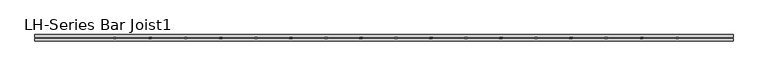
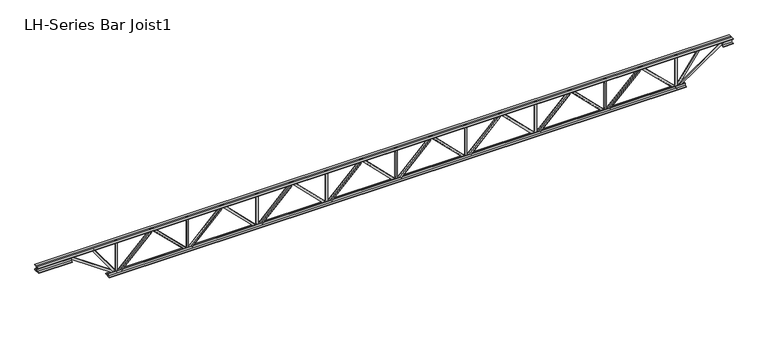
"""IFC4 building model written with IfcOpenShell, lengths in millimetres: beam geometry, LH-Series Bar Joist1 : 32LH-SP5."""

from ifc_helpers import new_model, si_unit, frame, origin, place, context, project, spatial, polyline, outline, extrude, faceted_brep, source, transform, mapped, element, save


def lh_series_bar_joist1_a0e3509c(model_context):
    return source(origin(), model_context, "Body", "SolidModel", [
        extrude(outline(polyline([(406.4, 3276.6), (406.4, 3225.8), (323.85, 3225.8), (312.7375, 3236.9125), (-312.7375, 3236.9125), (-323.85, 3225.8), (-406.4, 3225.8), (-406.4, 3276.6), (406.4, 3276.6)])), frame((0.0, -12.7, 0.0), z_axis=(0.0, 1.0, 0.0), x_axis=(0.0, 0.0, 1.0)), (0.0, 0.0, 1.0), 25.4),
        faceted_brep([(3251.2, 0.0, -355.6), (3251.2, 0.0, -406.4), (3251.2, 12.7, -406.4), (3251.2, 12.7, -355.6), (3236.3210245, 0.0, -355.6), (2474.3210245, 0.0, 406.4), (2413.0, 0.0, 406.4), (2413.0, 0.0, 355.6), (2453.2789755, 0.0, 355.6), (3215.2789755, 0.0, -406.4), (3215.2789755, 12.7, -406.4), (3151.7789755, 12.7, -342.9), (3160.7592316, 12.7, -333.9197439), (2474.9592316, 12.7, 351.8802561), (2465.9789755, 12.7, 342.9), (2453.2789755, 12.7, 355.6), (2413.0, 12.7, 355.6), (2413.0, 12.7, 406.4), (2474.3210245, 12.7, 406.4), (3236.3210245, 12.7, -355.6), (2465.9789755, 50.8, 342.9), (3151.7789755, 50.8, -342.9), (3160.7592316, 50.8, -333.9197439), (2474.9592316, 50.8, 351.8802561)], [[[0, 1, 2, 3]], [[1, 0, 4, 5, 6, 7, 8, 9]], [[2, 1, 9, 10]], [[3, 2, 10, 11, 12, 13, 14, 15, 16, 17, 18, 19]], [[0, 3, 19, 4]], [[9, 8, 15, 14, 20, 21, 11, 10]], [[5, 4, 19, 18]], [[7, 6, 17, 16]], [[8, 7, 16, 15]], [[6, 5, 18, 17]], [[11, 21, 22, 12]], [[13, 23, 20, 14]], [[22, 21, 20, 23]], [[12, 22, 23, 13]]]),
        faceted_brep([(1625.6, -12.7, -355.6), (1625.6, 0.0, -355.6), (1625.6, 0.0, -406.4), (1625.6, -12.7, -406.4), (1640.4789755, -12.7, -355.6), (1640.4789755, 0.0, -355.6), (2402.4789755, 0.0, 406.4), (2463.8, 0.0, 406.4), (2463.8, 0.0, 355.6), (2423.5210245, 0.0, 355.6), (1661.5210245, 0.0, -406.4), (1661.5210245, -12.7, -406.4), (1725.0210245, -12.7, -342.9), (1716.0407684, -12.7, -333.9197439), (2401.8407684, -12.7, 351.8802561), (2410.8210245, -12.7, 342.9), (2423.5210245, -12.7, 355.6), (2463.8, -12.7, 355.6), (2463.8, -12.7, 406.4), (2402.4789755, -12.7, 406.4), (2410.8210245, -50.8, 342.9), (1725.0210245, -50.8, -342.9), (1716.0407684, -50.8, -333.9197439), (2401.8407684, -50.8, 351.8802561)], [[[0, 1, 2, 3]], [[1, 0, 4, 5]], [[2, 1, 5, 6, 7, 8, 9, 10]], [[3, 2, 10, 11]], [[0, 3, 11, 12, 13, 14, 15, 16, 17, 18, 19, 4]], [[5, 4, 19, 6]], [[10, 9, 16, 15, 20, 21, 12, 11]], [[8, 7, 18, 17]], [[7, 6, 19, 18]], [[9, 8, 17, 16]], [[21, 22, 13, 12]], [[20, 15, 14, 23]], [[22, 21, 20, 23]], [[13, 22, 23, 14]]]),
        extrude(outline(polyline([(406.4, 1651.0), (406.4, 1600.2), (323.85, 1600.2), (312.7375, 1611.3125), (-312.7375, 1611.3125), (-323.85, 1600.2), (-406.4, 1600.2), (-406.4, 1651.0), (406.4, 1651.0)])), frame((0.0, -12.7, 0.0), z_axis=(0.0, 1.0, 0.0), x_axis=(0.0, 0.0, 1.0)), (0.0, 0.0, 1.0), 25.4),
        faceted_brep([(1625.6, 0.0, -355.6), (1625.6, 0.0, -406.4), (1625.6, 12.7, -406.4), (1625.6, 12.7, -355.6), (1610.7210245, 0.0, -355.6), (848.7210245, 0.0, 406.4), (787.4, 0.0, 406.4), (787.4, 0.0, 355.6), (827.6789755, 0.0, 355.6), (1589.6789755, 0.0, -406.4), (1589.6789755, 12.7, -406.4), (1526.1789755, 12.7, -342.9), (1535.1592316, 12.7, -333.9197439), (849.3592316, 12.7, 351.8802561), (840.3789755, 12.7, 342.9), (827.6789755, 12.7, 355.6), (787.4, 12.7, 355.6), (787.4, 12.7, 406.4), (848.7210245, 12.7, 406.4), (1610.7210245, 12.7, -355.6), (840.3789755, 50.8, 342.9), (1526.1789755, 50.8, -342.9), (1535.1592316, 50.8, -333.9197439), (849.3592316, 50.8, 351.8802561)], [[[0, 1, 2, 3]], [[1, 0, 4, 5, 6, 7, 8, 9]], [[2, 1, 9, 10]], [[3, 2, 10, 11, 12, 13, 14, 15, 16, 17, 18, 19]], [[0, 3, 19, 4]], [[9, 8, 15, 14, 20, 21, 11, 10]], [[5, 4, 19, 18]], [[7, 6, 17, 16]], [[8, 7, 16, 15]], [[6, 5, 18, 17]], [[11, 21, 22, 12]], [[13, 23, 20, 14]], [[22, 21, 20, 23]], [[12, 22, 23, 13]]]),
        faceted_brep([(0.0, -12.7, -355.6), (0.0, 0.0, -355.6), (0.0, 0.0, -406.4), (0.0, -12.7, -406.4), (14.8789755, -12.7, -355.6), (14.8789755, 0.0, -355.6), (776.8789755, 0.0, 406.4), (838.2, 0.0, 406.4), (838.2, 0.0, 355.6), (797.9210245, 0.0, 355.6), (35.9210245, 0.0, -406.4), (35.9210245, -12.7, -406.4), (99.4210245, -12.7, -342.9), (90.4407684, -12.7, -333.9197439), (776.2407684, -12.7, 351.8802561), (785.2210245, -12.7, 342.9), (797.9210245, -12.7, 355.6), (838.2, -12.7, 355.6), (838.2, -12.7, 406.4), (776.8789755, -12.7, 406.4), (785.2210245, -50.8, 342.9), (99.4210245, -50.8, -342.9), (90.4407684, -50.8, -333.9197439), (776.2407684, -50.8, 351.8802561)], [[[0, 1, 2, 3]], [[1, 0, 4, 5]], [[2, 1, 5, 6, 7, 8, 9, 10]], [[3, 2, 10, 11]], [[0, 3, 11, 12, 13, 14, 15, 16, 17, 18, 19, 4]], [[5, 4, 19, 6]], [[10, 9, 16, 15, 20, 21, 12, 11]], [[8, 7, 18, 17]], [[7, 6, 19, 18]], [[9, 8, 17, 16]], [[21, 22, 13, 12]], [[20, 15, 14, 23]], [[22, 21, 20, 23]], [[13, 22, 23, 14]]]),
        extrude(outline(polyline([(406.4, 25.4), (406.4, -25.4), (323.85, -25.4), (312.7375, -14.2875), (-312.7375, -14.2875), (-323.85, -25.4), (-406.4, -25.4), (-406.4, 25.4), (406.4, 25.4)])), frame((0.0, -12.7, 0.0), z_axis=(0.0, 1.0, 0.0), x_axis=(0.0, 0.0, 1.0)), (0.0, 0.0, 1.0), 25.4),
        faceted_brep([(0.0, 0.0, -355.6), (0.0, 0.0, -406.4), (0.0, 12.7, -406.4), (0.0, 12.7, -355.6), (-14.8789755, 0.0, -355.6), (-776.8789755, 0.0, 406.4), (-838.2, 0.0, 406.4), (-838.2, 0.0, 355.6), (-797.9210245, 0.0, 355.6), (-35.9210245, 0.0, -406.4), (-35.9210245, 12.7, -406.4), (-99.4210245, 12.7, -342.9), (-90.4407684, 12.7, -333.9197439), (-776.2407684, 12.7, 351.8802561), (-785.2210245, 12.7, 342.9), (-797.9210245, 12.7, 355.6), (-838.2, 12.7, 355.6), (-838.2, 12.7, 406.4), (-776.8789755, 12.7, 406.4), (-14.8789755, 12.7, -355.6), (-785.2210245, 50.8, 342.9), (-99.4210245, 50.8, -342.9), (-90.4407684, 50.8, -333.9197439), (-776.2407684, 50.8, 351.8802561)], [[[0, 1, 2, 3]], [[1, 0, 4, 5, 6, 7, 8, 9]], [[2, 1, 9, 10]], [[3, 2, 10, 11, 12, 13, 14, 15, 16, 17, 18, 19]], [[0, 3, 19, 4]], [[9, 8, 15, 14, 20, 21, 11, 10]], [[5, 4, 19, 18]], [[7, 6, 17, 16]], [[8, 7, 16, 15]], [[6, 5, 18, 17]], [[11, 21, 22, 12]], [[13, 23, 20, 14]], [[22, 21, 20, 23]], [[12, 22, 23, 13]]]),
        faceted_brep([(-1625.6, -12.7, -355.6), (-1625.6, 0.0, -355.6), (-1625.6, 0.0, -406.4), (-1625.6, -12.7, -406.4), (-1610.7210245, -12.7, -355.6), (-1610.7210245, 0.0, -355.6), (-848.7210245, 0.0, 406.4), (-787.4, 0.0, 406.4), (-787.4, 0.0, 355.6), (-827.6789755, 0.0, 355.6), (-1589.6789755, 0.0, -406.4), (-1589.6789755, -12.7, -406.4), (-1526.1789755, -12.7, -342.9), (-1535.1592316, -12.7, -333.9197439), (-849.3592316, -12.7, 351.8802561), (-840.3789755, -12.7, 342.9), (-827.6789755, -12.7, 355.6), (-787.4, -12.7, 355.6), (-787.4, -12.7, 406.4), (-848.7210245, -12.7, 406.4), (-840.3789755, -50.8, 342.9), (-1526.1789755, -50.8, -342.9), (-1535.1592316, -50.8, -333.9197439), (-849.3592316, -50.8, 351.8802561)], [[[0, 1, 2, 3]], [[1, 0, 4, 5]], [[2, 1, 5, 6, 7, 8, 9, 10]], [[3, 2, 10, 11]], [[0, 3, 11, 12, 13, 14, 15, 16, 17, 18, 19, 4]], [[5, 4, 19, 6]], [[10, 9, 16, 15, 20, 21, 12, 11]], [[8, 7, 18, 17]], [[7, 6, 19, 18]], [[9, 8, 17, 16]], [[21, 22, 13, 12]], [[20, 15, 14, 23]], [[22, 21, 20, 23]], [[13, 22, 23, 14]]]),
        extrude(outline(polyline([(406.4, 6556.375), (406.4, 6505.575), (323.85, 6505.575), (312.7375, 6516.6875), (-312.7375, 6516.6875), (-323.85, 6505.575), (-406.4, 6505.575), (-406.4, 6556.375), (406.4, 6556.375)])), frame((0.0, -12.7, 0.0), z_axis=(0.0, 1.0, 0.0), x_axis=(0.0, 0.0, 1.0)), (0.0, 0.0, 1.0), 25.4),
        faceted_brep([(6530.975, 0.0, -355.6), (6530.975, 0.0, -406.4), (6530.975, 12.7, -406.4), (6530.975, 12.7, -355.6), (6515.958098, 0.0, -355.6), (5739.670598, 0.0, 406.4), (5678.4875, 0.0, 406.4), (5678.4875, 0.0, 355.6), (5718.904402, 0.0, 355.6), (6495.191902, 0.0, -406.4), (6495.191902, 12.7, -406.4), (6431.104883, 12.7, -343.4924966), (6440.0013474, 12.7, -334.4292234), (5740.6182703, 12.7, 352.0817725), (5731.7218059, 12.7, 343.0184993), (5718.904402, 12.7, 355.6), (5678.4875, 12.7, 355.6), (5678.4875, 12.7, 406.4), (5739.670598, 12.7, 406.4), (6515.958098, 12.7, -355.6), (5731.7218059, 50.8, 343.0184993), (6431.104883, 50.8, -343.4924966), (6440.0013474, 50.8, -334.4292234), (5740.6182703, 50.8, 352.0817725)], [[[0, 1, 2, 3]], [[1, 0, 4, 5, 6, 7, 8, 9]], [[2, 1, 9, 10]], [[3, 2, 10, 11, 12, 13, 14, 15, 16, 17, 18, 19]], [[0, 3, 19, 4]], [[9, 8, 15, 14, 20, 21, 11, 10]], [[5, 4, 19, 18]], [[7, 6, 17, 16]], [[8, 7, 16, 15]], [[6, 5, 18, 17]], [[11, 21, 22, 12]], [[13, 23, 20, 14]], [[22, 21, 20, 23]], [[12, 22, 23, 13]]]),
        faceted_brep([(4876.8, -12.7, -355.6), (4876.8, 0.0, -355.6), (4876.8, 0.0, -406.4), (4876.8, -12.7, -406.4), (4891.816902, -12.7, -355.6), (4891.816902, 0.0, -355.6), (5668.104402, 0.0, 406.4), (5729.2875, 0.0, 406.4), (5729.2875, 0.0, 355.6), (5688.870598, 0.0, 355.6), (4912.583098, 0.0, -406.4), (4912.583098, -12.7, -406.4), (4976.670117, -12.7, -343.4924966), (4967.7736526, -12.7, -334.4292234), (5667.1567297, -12.7, 352.0817725), (5676.0531941, -12.7, 343.0184993), (5688.870598, -12.7, 355.6), (5729.2875, -12.7, 355.6), (5729.2875, -12.7, 406.4), (5668.104402, -12.7, 406.4), (5676.0531941, -50.8, 343.0184993), (4976.670117, -50.8, -343.4924966), (4967.7736526, -50.8, -334.4292234), (5667.1567297, -50.8, 352.0817725)], [[[0, 1, 2, 3]], [[1, 0, 4, 5]], [[2, 1, 5, 6, 7, 8, 9, 10]], [[3, 2, 10, 11]], [[0, 3, 11, 12, 13, 14, 15, 16, 17, 18, 19, 4]], [[5, 4, 19, 6]], [[10, 9, 16, 15, 20, 21, 12, 11]], [[8, 7, 18, 17]], [[7, 6, 19, 18]], [[9, 8, 17, 16]], [[21, 22, 13, 12]], [[20, 15, 14, 23]], [[22, 21, 20, 23]], [[13, 22, 23, 14]]]),
        extrude(outline(polyline([(406.4, -4851.4), (406.4, -4902.2), (323.85, -4902.2), (312.7375, -4891.0875), (-312.7375, -4891.0875), (-323.85, -4902.2), (-406.4, -4902.2), (-406.4, -4851.4), (406.4, -4851.4)])), frame((0.0, -12.7, 0.0), z_axis=(0.0, 1.0, 0.0), x_axis=(0.0, 0.0, 1.0)), (0.0, 0.0, 1.0), 25.4),
        extrude(outline(polyline([(406.4, -6505.575), (406.4, -6556.375), (323.85, -6556.375), (312.7375, -6545.2625), (-312.7375, -6545.2625), (-323.85, -6556.375), (-406.4, -6556.375), (-406.4, -6505.575), (406.4, -6505.575)])), frame((0.0, -12.7, 0.0), z_axis=(0.0, 1.0, 0.0), x_axis=(0.0, 0.0, 1.0)), (0.0, 0.0, 1.0), 25.4),
        faceted_brep([(-4876.8, 0.0, -355.6), (-4876.8, 0.0, -406.4), (-4876.8, 12.7, -406.4), (-4876.8, 12.7, -355.6), (-4891.816902, 0.0, -355.6), (-5668.104402, 0.0, 406.4), (-5729.2875, 0.0, 406.4), (-5729.2875, 0.0, 355.6), (-5688.870598, 0.0, 355.6), (-4912.583098, 0.0, -406.4), (-4912.583098, 12.7, -406.4), (-4976.670117, 12.7, -343.4924966), (-4967.7736526, 12.7, -334.4292234), (-5667.1567297, 12.7, 352.0817725), (-5676.0531941, 12.7, 343.0184993), (-5688.870598, 12.7, 355.6), (-5729.2875, 12.7, 355.6), (-5729.2875, 12.7, 406.4), (-5668.104402, 12.7, 406.4), (-4891.816902, 12.7, -355.6), (-5676.0531941, 50.8, 343.0184993), (-4976.670117, 50.8, -343.4924966), (-4967.7736526, 50.8, -334.4292234), (-5667.1567297, 50.8, 352.0817725)], [[[0, 1, 2, 3]], [[1, 0, 4, 5, 6, 7, 8, 9]], [[2, 1, 9, 10]], [[3, 2, 10, 11, 12, 13, 14, 15, 16, 17, 18, 19]], [[0, 3, 19, 4]], [[9, 8, 15, 14, 20, 21, 11, 10]], [[5, 4, 19, 18]], [[7, 6, 17, 16]], [[8, 7, 16, 15]], [[6, 5, 18, 17]], [[11, 21, 22, 12]], [[13, 23, 20, 14]], [[22, 21, 20, 23]], [[12, 22, 23, 13]]]),
        faceted_brep([(-6530.975, -12.7, -355.6), (-6530.975, 0.0, -355.6), (-6530.975, 0.0, -406.4), (-6530.975, -12.7, -406.4), (-6515.958098, -12.7, -355.6), (-6515.958098, 0.0, -355.6), (-5739.670598, 0.0, 406.4), (-5678.4875, 0.0, 406.4), (-5678.4875, 0.0, 355.6), (-5718.904402, 0.0, 355.6), (-6495.191902, 0.0, -406.4), (-6495.191902, -12.7, -406.4), (-6431.104883, -12.7, -343.4924966), (-6440.0013474, -12.7, -334.4292234), (-5740.6182703, -12.7, 352.0817725), (-5731.7218059, -12.7, 343.0184993), (-5718.904402, -12.7, 355.6), (-5678.4875, -12.7, 355.6), (-5678.4875, -12.7, 406.4), (-5739.670598, -12.7, 406.4), (-5731.7218059, -50.8, 343.0184993), (-6431.104883, -50.8, -343.4924966), (-6440.0013474, -50.8, -334.4292234), (-5740.6182703, -50.8, 352.0817725)], [[[0, 1, 2, 3]], [[1, 0, 4, 5]], [[2, 1, 5, 6, 7, 8, 9, 10]], [[3, 2, 10, 11]], [[0, 3, 11, 12, 13, 14, 15, 16, 17, 18, 19, 4]], [[5, 4, 19, 6]], [[10, 9, 16, 15, 20, 21, 12, 11]], [[8, 7, 18, 17]], [[7, 6, 19, 18]], [[9, 8, 17, 16]], [[21, 22, 13, 12]], [[20, 15, 14, 23]], [[22, 21, 20, 23]], [[13, 22, 23, 14]]]),
        extrude(outline(polyline([(406.4, -1600.2), (406.4, -1651.0), (323.85, -1651.0), (312.7375, -1639.8875), (-312.7375, -1639.8875), (-323.85, -1651.0), (-406.4, -1651.0), (-406.4, -1600.2), (406.4, -1600.2)])), frame((0.0, -12.7, 0.0), z_axis=(0.0, 1.0, 0.0), x_axis=(0.0, 0.0, 1.0)), (0.0, 0.0, 1.0), 25.4),
        faceted_brep([(-1625.6, 0.0, -355.6), (-1625.6, 0.0, -406.4), (-1625.6, 12.7, -406.4), (-1625.6, 12.7, -355.6), (-1640.4789755, 0.0, -355.6), (-2402.4789755, 0.0, 406.4), (-2463.8, 0.0, 406.4), (-2463.8, 0.0, 355.6), (-2423.5210245, 0.0, 355.6), (-1661.5210245, 0.0, -406.4), (-1661.5210245, 12.7, -406.4), (-1725.0210245, 12.7, -342.9), (-1716.0407684, 12.7, -333.9197439), (-2401.8407684, 12.7, 351.8802561), (-2410.8210245, 12.7, 342.9), (-2423.5210245, 12.7, 355.6), (-2463.8, 12.7, 355.6), (-2463.8, 12.7, 406.4), (-2402.4789755, 12.7, 406.4), (-1640.4789755, 12.7, -355.6), (-2410.8210245, 50.8, 342.9), (-1725.0210245, 50.8, -342.9), (-1716.0407684, 50.8, -333.9197439), (-2401.8407684, 50.8, 351.8802561)], [[[0, 1, 2, 3]], [[1, 0, 4, 5, 6, 7, 8, 9]], [[2, 1, 9, 10]], [[3, 2, 10, 11, 12, 13, 14, 15, 16, 17, 18, 19]], [[0, 3, 19, 4]], [[9, 8, 15, 14, 20, 21, 11, 10]], [[5, 4, 19, 18]], [[7, 6, 17, 16]], [[8, 7, 16, 15]], [[6, 5, 18, 17]], [[11, 21, 22, 12]], [[13, 23, 20, 14]], [[22, 21, 20, 23]], [[12, 22, 23, 13]]]),
        faceted_brep([(-3251.2, -12.7, -355.6), (-3251.2, 0.0, -355.6), (-3251.2, 0.0, -406.4), (-3251.2, -12.7, -406.4), (-3236.3210245, -12.7, -355.6), (-3236.3210245, 0.0, -355.6), (-2474.3210245, 0.0, 406.4), (-2413.0, 0.0, 406.4), (-2413.0, 0.0, 355.6), (-2453.2789755, 0.0, 355.6), (-3215.2789755, 0.0, -406.4), (-3215.2789755, -12.7, -406.4), (-3151.7789755, -12.7, -342.9), (-3160.7592316, -12.7, -333.9197439), (-2474.9592316, -12.7, 351.8802561), (-2465.9789755, -12.7, 342.9), (-2453.2789755, -12.7, 355.6), (-2413.0, -12.7, 355.6), (-2413.0, -12.7, 406.4), (-2474.3210245, -12.7, 406.4), (-2465.9789755, -50.8, 342.9), (-3151.7789755, -50.8, -342.9), (-3160.7592316, -50.8, -333.9197439), (-2474.9592316, -50.8, 351.8802561)], [[[0, 1, 2, 3]], [[1, 0, 4, 5]], [[2, 1, 5, 6, 7, 8, 9, 10]], [[3, 2, 10, 11]], [[0, 3, 11, 12, 13, 14, 15, 16, 17, 18, 19, 4]], [[5, 4, 19, 6]], [[10, 9, 16, 15, 20, 21, 12, 11]], [[8, 7, 18, 17]], [[7, 6, 19, 18]], [[9, 8, 17, 16]], [[21, 22, 13, 12]], [[20, 15, 14, 23]], [[22, 21, 20, 23]], [[13, 22, 23, 14]]]),
        extrude(outline(polyline([(406.4, 4902.2), (406.4, 4851.4), (323.85, 4851.4), (312.7375, 4862.5125), (-312.7375, 4862.5125), (-323.85, 4851.4), (-406.4, 4851.4), (-406.4, 4902.2), (406.4, 4902.2)])), frame((0.0, -12.7, 0.0), z_axis=(0.0, 1.0, 0.0), x_axis=(0.0, 0.0, 1.0)), (0.0, 0.0, 1.0), 25.4),
        faceted_brep([(4876.8, 0.0, -355.6), (4876.8, 0.0, -406.4), (4876.8, 12.7, -406.4), (4876.8, 12.7, -355.6), (4861.9210245, 0.0, -355.6), (4099.9210245, 0.0, 406.4), (4038.6, 0.0, 406.4), (4038.6, 0.0, 355.6), (4078.8789755, 0.0, 355.6), (4840.8789755, 0.0, -406.4), (4840.8789755, 12.7, -406.4), (4777.3789755, 12.7, -342.9), (4786.3592316, 12.7, -333.9197439), (4100.5592316, 12.7, 351.8802561), (4091.5789755, 12.7, 342.9), (4078.8789755, 12.7, 355.6), (4038.6, 12.7, 355.6), (4038.6, 12.7, 406.4), (4099.9210245, 12.7, 406.4), (4861.9210245, 12.7, -355.6), (4091.5789755, 50.8, 342.9), (4777.3789755, 50.8, -342.9), (4786.3592316, 50.8, -333.9197439), (4100.5592316, 50.8, 351.8802561)], [[[0, 1, 2, 3]], [[1, 0, 4, 5, 6, 7, 8, 9]], [[2, 1, 9, 10]], [[3, 2, 10, 11, 12, 13, 14, 15, 16, 17, 18, 19]], [[0, 3, 19, 4]], [[9, 8, 15, 14, 20, 21, 11, 10]], [[5, 4, 19, 18]], [[7, 6, 17, 16]], [[8, 7, 16, 15]], [[6, 5, 18, 17]], [[11, 21, 22, 12]], [[13, 23, 20, 14]], [[22, 21, 20, 23]], [[12, 22, 23, 13]]]),
        faceted_brep([(3251.2, -12.7, -355.6), (3251.2, 0.0, -355.6), (3251.2, 0.0, -406.4), (3251.2, -12.7, -406.4), (3266.0789755, -12.7, -355.6), (3266.0789755, 0.0, -355.6), (4028.0789755, 0.0, 406.4), (4089.4, 0.0, 406.4), (4089.4, 0.0, 355.6), (4049.1210245, 0.0, 355.6), (3287.1210245, 0.0, -406.4), (3287.1210245, -12.7, -406.4), (3350.6210245, -12.7, -342.9), (3341.6407684, -12.7, -333.9197439), (4027.4407684, -12.7, 351.8802561), (4036.4210245, -12.7, 342.9), (4049.1210245, -12.7, 355.6), (4089.4, -12.7, 355.6), (4089.4, -12.7, 406.4), (4028.0789755, -12.7, 406.4), (4036.4210245, -50.8, 342.9), (3350.6210245, -50.8, -342.9), (3341.6407684, -50.8, -333.9197439), (4027.4407684, -50.8, 351.8802561)], [[[0, 1, 2, 3]], [[1, 0, 4, 5]], [[2, 1, 5, 6, 7, 8, 9, 10]], [[3, 2, 10, 11]], [[0, 3, 11, 12, 13, 14, 15, 16, 17, 18, 19, 4]], [[5, 4, 19, 6]], [[10, 9, 16, 15, 20, 21, 12, 11]], [[8, 7, 18, 17]], [[7, 6, 19, 18]], [[9, 8, 17, 16]], [[21, 22, 13, 12]], [[20, 15, 14, 23]], [[22, 21, 20, 23]], [[13, 22, 23, 14]]]),
        extrude(outline(polyline([(406.4, -3225.8), (406.4, -3276.6), (323.85, -3276.6), (312.7375, -3265.4875), (-312.7375, -3265.4875), (-323.85, -3276.6), (-406.4, -3276.6), (-406.4, -3225.8), (406.4, -3225.8)])), frame((0.0, -12.7, 0.0), z_axis=(0.0, 1.0, 0.0), x_axis=(0.0, 0.0, 1.0)), (0.0, 0.0, 1.0), 25.4),
        faceted_brep([(-3251.2, 0.0, -355.6), (-3251.2, 0.0, -406.4), (-3251.2, 12.7, -406.4), (-3251.2, 12.7, -355.6), (-3266.0789755, 0.0, -355.6), (-4028.0789755, 0.0, 406.4), (-4089.4, 0.0, 406.4), (-4089.4, 0.0, 355.6), (-4049.1210245, 0.0, 355.6), (-3287.1210245, 0.0, -406.4), (-3287.1210245, 12.7, -406.4), (-3350.6210245, 12.7, -342.9), (-3341.6407684, 12.7, -333.9197439), (-4027.4407684, 12.7, 351.8802561), (-4036.4210245, 12.7, 342.9), (-4049.1210245, 12.7, 355.6), (-4089.4, 12.7, 355.6), (-4089.4, 12.7, 406.4), (-4028.0789755, 12.7, 406.4), (-3266.0789755, 12.7, -355.6), (-4036.4210245, 50.8, 342.9), (-3350.6210245, 50.8, -342.9), (-3341.6407684, 50.8, -333.9197439), (-4027.4407684, 50.8, 351.8802561)], [[[0, 1, 2, 3]], [[1, 0, 4, 5, 6, 7, 8, 9]], [[2, 1, 9, 10]], [[3, 2, 10, 11, 12, 13, 14, 15, 16, 17, 18, 19]], [[0, 3, 19, 4]], [[9, 8, 15, 14, 20, 21, 11, 10]], [[5, 4, 19, 18]], [[7, 6, 17, 16]], [[8, 7, 16, 15]], [[6, 5, 18, 17]], [[11, 21, 22, 12]], [[13, 23, 20, 14]], [[22, 21, 20, 23]], [[12, 22, 23, 13]]]),
        faceted_brep([(-4876.8, -12.7, -355.6), (-4876.8, 0.0, -355.6), (-4876.8, 0.0, -406.4), (-4876.8, -12.7, -406.4), (-4861.9210245, -12.7, -355.6), (-4861.9210245, 0.0, -355.6), (-4099.9210245, 0.0, 406.4), (-4038.6, 0.0, 406.4), (-4038.6, 0.0, 355.6), (-4078.8789755, 0.0, 355.6), (-4840.8789755, 0.0, -406.4), (-4840.8789755, -12.7, -406.4), (-4777.3789755, -12.7, -342.9), (-4786.3592316, -12.7, -333.9197439), (-4100.5592316, -12.7, 351.8802561), (-4091.5789755, -12.7, 342.9), (-4078.8789755, -12.7, 355.6), (-4038.6, -12.7, 355.6), (-4038.6, -12.7, 406.4), (-4099.9210245, -12.7, 406.4), (-4091.5789755, -50.8, 342.9), (-4777.3789755, -50.8, -342.9), (-4786.3592316, -50.8, -333.9197439), (-4100.5592316, -50.8, 351.8802561)], [[[0, 1, 2, 3]], [[1, 0, 4, 5]], [[2, 1, 5, 6, 7, 8, 9, 10]], [[3, 2, 10, 11]], [[0, 3, 11, 12, 13, 14, 15, 16, 17, 18, 19, 4]], [[5, 4, 19, 6]], [[10, 9, 16, 15, 20, 21, 12, 11]], [[8, 7, 18, 17]], [[7, 6, 19, 18]], [[9, 8, 17, 16]], [[21, 22, 13, 12]], [[20, 15, 14, 23]], [[22, 21, 20, 23]], [[13, 22, 23, 14]]]),
        extrude(outline(polyline([(12.7, 406.4), (76.2, 406.4), (76.2, 393.7), (25.4, 393.7), (25.4, 342.9), (12.7, 342.9), (12.7, 406.4)])), frame((-8381.9219944, 0.0, 0.0), z_axis=(1.0, 0.0, 0.0), x_axis=(0.0, 1.0, 0.0)), (0.0, 0.0, 1.0), 16208.2969944),
        extrude(outline(polyline([(-12.7, 406.4), (-12.7, 342.9), (-25.4, 342.9), (-25.4, 393.7), (-76.2, 393.7), (-76.2, 406.4), (-12.7, 406.4)])), frame((-8381.9219944, 0.0, 0.0), z_axis=(1.0, 0.0, 0.0), x_axis=(0.0, 1.0, 0.0)), (0.0, 0.0, 1.0), 16208.2969944),
        extrude(outline(polyline([(-12.7, 279.4), (-76.2, 279.4), (-76.2, 292.1), (-25.4, 292.1), (-25.4, 342.9), (-12.7, 342.9), (-12.7, 279.4)])), frame((-8381.9219944, 0.0, 0.0), z_axis=(1.0, 0.0, 0.0), x_axis=(0.0, 1.0, 0.0)), (0.0, 0.0, 1.0), 784.1469944),
        extrude(outline(polyline([(76.2, 279.4), (12.7, 279.4), (12.7, 342.9), (25.4, 342.9), (25.4, 292.1), (76.2, 292.1), (76.2, 279.4)])), frame((-8381.9219944, 0.0, 0.0), z_axis=(1.0, 0.0, 0.0), x_axis=(0.0, 1.0, 0.0)), (0.0, 0.0, 1.0), 784.1469944),
        extrude(outline(polyline([(12.7, 279.4), (12.7, 342.9), (25.4, 342.9), (25.4, 292.1), (76.2, 292.1), (76.2, 279.4), (12.7, 279.4)])), frame((7597.775, 0.0, 0.0), z_axis=(1.0, 0.0, 0.0), x_axis=(0.0, 1.0, 0.0)), (0.0, 0.0, 1.0), 228.6),
        extrude(outline(polyline([(-12.7, 279.4), (-76.2, 279.4), (-76.2, 292.1), (-25.4, 292.1), (-25.4, 342.9), (-12.7, 342.9), (-12.7, 279.4)])), frame((7597.775, 0.0, 0.0), z_axis=(1.0, 0.0, 0.0), x_axis=(0.0, 1.0, 0.0)), (0.0, 0.0, 1.0), 228.6),
        extrude(outline(polyline([(12.7, -406.4), (12.7, -342.9), (25.4, -342.9), (25.4, -393.7), (76.2, -393.7), (76.2, -406.4), (12.7, -406.4)])), frame((-6734.175, 0.0, 0.0), z_axis=(1.0, 0.0, 0.0), x_axis=(0.0, 1.0, 0.0)), (0.0, 0.0, 1.0), 13468.35),
        extrude(outline(polyline([(-12.7, -406.4), (-76.2, -406.4), (-76.2, -393.7), (-25.4, -393.7), (-25.4, -342.9), (-12.7, -342.9), (-12.7, -406.4)])), frame((-6734.175, 0.0, 0.0), z_axis=(1.0, 0.0, 0.0), x_axis=(0.0, 1.0, 0.0)), (0.0, 0.0, 1.0), 13468.35),
        extrude(outline(polyline([(6.35, -25.4), (-6.35, -25.4), (-6.35, 25.4), (6.35, 25.4), (6.35, -25.4)])), frame((-6530.975, 0.0, -400.05), z_axis=(-0.58320678309139, 0.0, 0.8123237335915974), x_axis=(0.0, -1.0, 0.0)), (0.0, 0.0, 1.0), 914.598416),
        extrude(outline(polyline([(0.0, -12.7), (0.0, 0.0), (1300.0142086, 0.0), (1300.0142086, -12.7), (0.0, -12.7)])), frame((-7612.2909413, 6.35, 322.056597), z_axis=(0.5714937537595753, 0.0, 0.8206064156547828), x_axis=(0.8206064156547828, 0.0, -0.5714937537595753)), (0.0, 0.0, 1.0), 50.8),
        extrude(outline(polyline([(6.35, 25.4), (6.35, -25.4), (-6.35, -25.4), (-6.35, 25.4), (6.35, 25.4)])), frame((6530.975, 0.0, -400.05), z_axis=(0.5811065900870399, 0.0, 0.8138274577313137), x_axis=(0.0, -1.0, 0.0)), (0.0, 0.0, 1.0), 912.9084955),
        extrude(outline(polyline([(0.0, -12.7), (0.0, 0.0), (1300.0142086, 0.0), (1300.0142086, -12.7), (0.0, -12.7)])), frame((6545.4909413, -6.35, -420.893403), z_axis=(-0.5714937537593278, 0.0, 0.8206064156549552), x_axis=(0.8206064156549552, 0.0, 0.5714937537593278)), (0.0, 0.0, 1.0), 50.8),
    ])


if __name__ == "__main__":
    model = new_model("IFC4")
    model_context = context("Model", 3, world=origin())
    ifc_project = project(units=[si_unit("LENGTHUNIT", "METRE", prefix="MILLI")], contexts=[model_context])
    site = spatial("IfcSite", under=ifc_project)
    building = spatial("IfcBuilding", under=site)
    placement = place(None, origin())
    lh_series_bar_joist1_shape = lh_series_bar_joist1_a0e3509c(model_context)
    element("IfcBeam", 1, ObjectType="LH-Series Bar Joist1 : 32LH-SP5", at=placement, inside=building, context=model_context, shape_type="MappedRepresentation", body=[
        mapped(lh_series_bar_joist1_shape, transform((0.0, 0.0, 0.0), x_axis=(1.0, 0.0, 0.0), y_axis=(0.0, 1.0, 0.0), z_axis=(0.0, 0.0, 1.0))),
    ])
    save(model, "model.ifc")

# Revit data of these elements
# Type "LH-Series Bar Joist1 : 32LH-SP5"
#   Assembly Code = "B1010350"
#   Wt = 30
#   Web Thickness = 0' - 1"
#   Variable Panel [instance default] = 5' - 4"
#   Start Offset [instance default] = 0' - 0"
#   Start Extension [instance default] = 0' - 0"
#   Seat Length = 0' - 6"
#   Seat Depth = 0' - 5"
#   IntPanelWidth [instance default] = 5' - 4"
#   IntPanelArrayLength [instance default] = 21' - 4"
#   PanelAreaLength [instance default] = 32' - 0"
#   End Panel = 4' - 0"
#   End Offset [instance default] = 0' - 0"
#   End Extension [instance default] = 0' - 0"
#   Cord Leg = 0' - 2 1/2"
#   Chord Thickness = 0' - 0 1/2"
#   Length [instance default] = 40' - 0"
#   Depth = 2' - 8"
#   Vertical Member Visibility = yes
#   IntPanelArrayNum [instance default] = 4
#   Structural Material = none
# Element 1 (IfcBeam, "LH-Series Bar Joist1 : 32LH-SP5")
#   Variable Panel = 5' - 5 1/8"
#   Start Extension = 2' - 0.87193"
#   IntPanelArrayLength = 32' - 0"
#   PanelAreaLength = 42' - 10 1/4"
#   End Extension = 0' - 3"
#   Length = 50' - 10 1/4"
#   IntPanelArrayNum = 6
